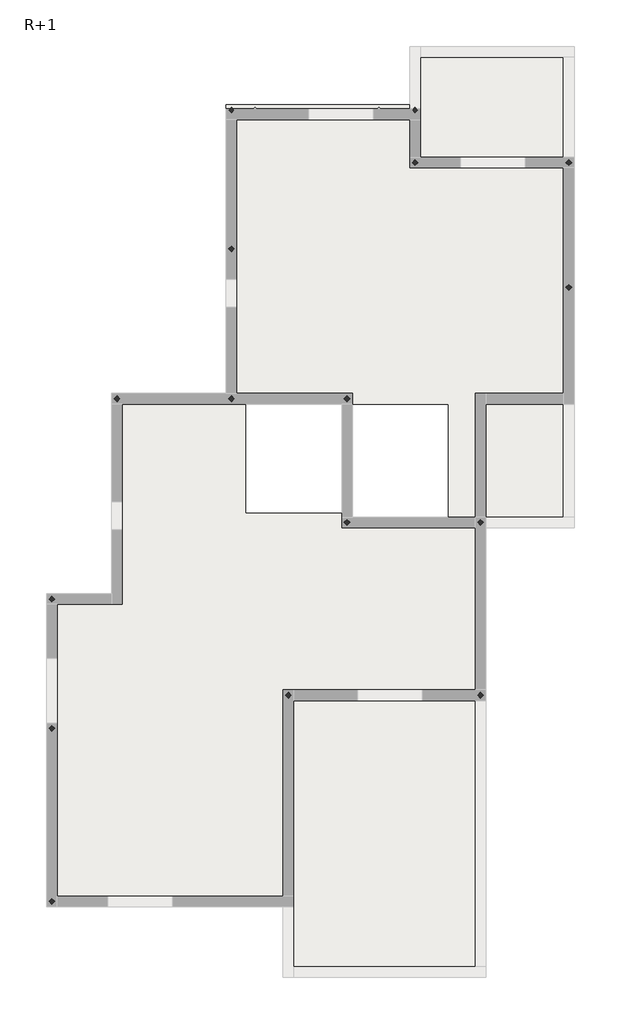
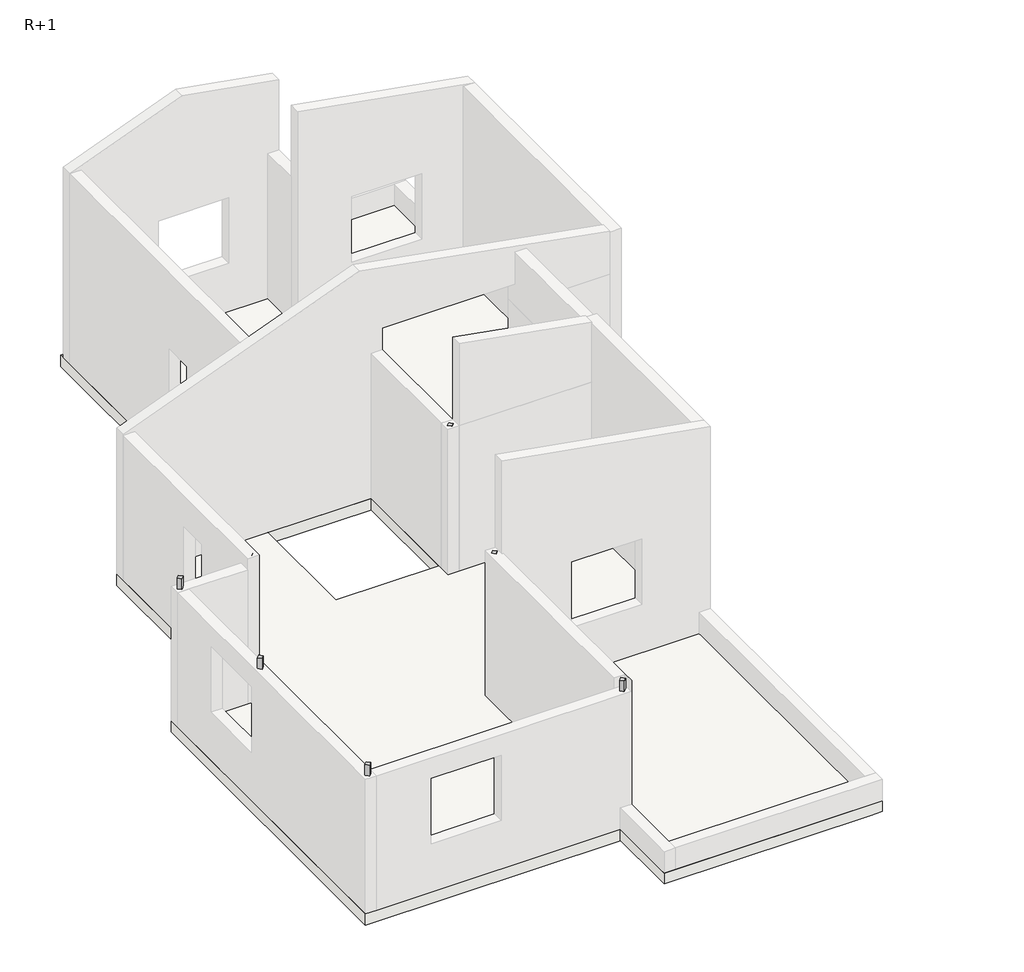
# One storey, part 2 of 2: 20 columns, 4 slabs, 1 beam.
"""IFC4 building model written with IfcOpenShell, lengths in millimetres."""

import ifcopenshell
import ifcopenshell.guid

model = None  # the IFC model being written
_history = None  # IfcOwnerHistory: only IFC2X3 demands one
_inside = {}  # id of a spatial element -> (the spatial element, [elements in it])
_under = {}  # id of a project, library or spatial element -> (it, [spatial elements below it])
_declared = {}  # id of a project -> (the project, [libraries it declares])
_typed = {}  # id of a type object -> (the type object, [elements of that type])
_made_of = {}  # id of a material, layer set ... -> (it, [elements and type objects made of it])


def new_model(schema):
    """Start an empty IFC model of exactly this schema.

    Asked for "IFC4X3", IfcOpenShell would pick the latest addendum, in which some entities
    have other attributes; the version numbers below select the first issue.
    IFC2X3 requires an IfcOwnerHistory on every rooted entity: one is made here for all.
    """
    global model, _history
    if schema == "IFC4X3":
        model = ifcopenshell.file(schema_version=(4, 3, 0, 0))
    else:
        model = ifcopenshell.file(schema=schema)
    _inside.clear()
    _under.clear()
    _declared.clear()
    _typed.clear()
    _made_of.clear()
    _history = None
    if model.schema == "IFC2X3":
        org = make("IfcOrganization", Name="unknown")
        user = make(
            "IfcPersonAndOrganization",
            ThePerson=make("IfcPerson", FamilyName="unknown"),
            TheOrganization=org,
        )
        app = make(
            "IfcApplication",
            ApplicationDeveloper=org,
            Version="unknown",
            ApplicationFullName="unknown",
            ApplicationIdentifier="unknown",
        )
        _history = make(
            "IfcOwnerHistory",
            OwningUser=user,
            OwningApplication=app,
            ChangeAction="ADDED",
            CreationDate=0,
        )
    return model


def make(cls, **values):
    """One entity of the class cls with the attributes given. An attribute that is None is left unset."""
    return model.create_entity(
        cls, **{name: value for name, value in values.items() if value is not None}
    )


def rooted(cls, **values):
    """An entity with a GlobalId (a new one), such as an element, a storey or a relation."""
    return make(cls, GlobalId=ifcopenshell.guid.new(), OwnerHistory=_history, **values)


def si_unit(unit_type, name, prefix=None):
    """IfcSIUnit, for example si_unit("LENGTHUNIT", "METRE", prefix="MILLI")."""
    return make("IfcSIUnit", UnitType=unit_type, Prefix=prefix, Name=name)


def assignment(units):
    """IfcUnitAssignment: the units of a project."""
    return None if units is None else make("IfcUnitAssignment", Units=units)


def point(xyz):
    """IfcCartesianPoint."""
    return None if xyz is None else make("IfcCartesianPoint", Coordinates=xyz)


def direction(xyz):
    """IfcDirection."""
    return None if xyz is None else make("IfcDirection", DirectionRatios=xyz)


def frame(location, z_axis=None, x_axis=None):
    """IfcAxis2Placement3D, a coordinate frame: its origin and axes. An axis left out is left unset."""
    return make(
        "IfcAxis2Placement3D",
        Location=point(location),
        Axis=direction(z_axis),
        RefDirection=direction(x_axis),
    )


def origin():
    """The frame at (0, 0, 0) with its axes left unset."""
    return frame((0.0, 0.0, 0.0))


def place(relative_to, where):
    """IfcLocalPlacement: puts the frame where relative to a parent placement (None: the world)."""
    return make(
        "IfcLocalPlacement", PlacementRelTo=relative_to, RelativePlacement=where
    )


def context(
    kind, dimensions, precision=None, world=None, true_north=None, identifier=None
):
    """IfcGeometricRepresentationContext, for example the 3D "Model" context."""
    return make(
        "IfcGeometricRepresentationContext",
        ContextIdentifier=identifier,
        ContextType=kind,
        CoordinateSpaceDimension=dimensions,
        Precision=precision,
        WorldCoordinateSystem=world,
        TrueNorth=true_north,
    )


def project(units=None, contexts=None):
    """IfcProject with its units and contexts."""
    return rooted(
        "IfcProject",
        Name="project",
        RepresentationContexts=contexts,
        UnitsInContext=assignment(units),
    )


def spatial(cls, under=None, at=None, **own):
    """A site, building, storey or space (cls), placed at a placement, below another one or the project."""
    s = rooted(cls, ObjectPlacement=at, **own)
    if under is not None:
        _under.setdefault(under.id(), (under, []))[1].append(s)
    return s


def polyline(points):
    """IfcPolyline through the points."""
    return make("IfcPolyline", Points=[point(p) for p in points])


def outline(outer, holes=None, kind="AREA"):
    """IfcArbitraryClosedProfileDef: a profile drawn as a closed curve; with holes, ...WithVoids."""
    if holes is None:
        return make("IfcArbitraryClosedProfileDef", ProfileType=kind, OuterCurve=outer)
    return make(
        "IfcArbitraryProfileDefWithVoids",
        ProfileType=kind,
        OuterCurve=outer,
        InnerCurves=holes,
    )


def extrude(swept, where, along, depth):
    """IfcExtrudedAreaSolid: the profile swept, set in the frame where, extruded along a direction by depth."""
    return make(
        "IfcExtrudedAreaSolid",
        SweptArea=swept,
        Position=where,
        ExtrudedDirection=direction(along),
        Depth=depth,
    )


def faces_of(points, faces, orient=None, outer=None):
    """IfcFace entities. A face is a list of loops; a loop is a list of indices into points, from 0.

    orient and outer hold one flag for each loop. By default every Orientation is true, the
    first loop of a face is its IfcFaceOuterBound and the others are IfcFaceBound.
    """
    made = []
    for i, loops in enumerate(faces):
        bounds = []
        for j, loop in enumerate(loops):
            is_outer = j == 0 if outer is None else outer[i][j]
            bounds.append(
                make(
                    "IfcFaceOuterBound" if is_outer else "IfcFaceBound",
                    Bound=make("IfcPolyLoop", Polygon=[points[k] for k in loop]),
                    Orientation=True if orient is None else orient[i][j],
                )
            )
        made.append(make("IfcFace", Bounds=bounds))
    return made


def faceted_brep(points, faces, orient=None, outer=None, voids=None):
    """IfcFacetedBrep: a solid bounded by flat faces; with voids (closed shells), ...WithVoids."""
    shared = [point(p) for p in points]
    hull = make("IfcClosedShell", CfsFaces=faces_of(shared, faces, orient, outer))
    if voids is None:
        return make("IfcFacetedBrep", Outer=hull)
    return make(
        "IfcFacetedBrepWithVoids",
        Outer=hull,
        Voids=[
            make(cls, CfsFaces=faces_of(shared, fs, o, b)) for cls, fs, o, b in voids
        ],
    )


def shape(context_of_items, identifier, shape_type, items):
    """IfcShapeRepresentation: the items that make up one representation, for example the "Body"."""
    return make(
        "IfcShapeRepresentation",
        ContextOfItems=context_of_items,
        RepresentationIdentifier=identifier,
        RepresentationType=shape_type,
        Items=items,
    )


def made_of(thing, what):
    """Note that an element or type object is made of a material, layer set ...; save() writes the relation."""
    if what is not None:
        _made_of.setdefault(what.id(), (what, []))[1].append(thing)
    return thing


def element(
    cls,
    number,
    at=None,
    inside=None,
    cuts=None,
    type_object=None,
    material=None,
    context=None,
    identifier="Body",
    shape_type=None,
    held_by="IfcProductDefinitionShape",
    body=None,
    shapes=None,
    **own,
):
    """One element of the class cls, such as IfcWall. Its Tag is "e" and its number.

    at: its placement. inside: the storey or other place that contains it. cuts: it is an
    opening in that element (IfcRelVoidsElement). A single representation is given by context,
    identifier, shape_type and body (its items); several are given by shapes. held_by: the class
    of the entity that holds the representations. save() writes the other relations.
    """
    e = rooted(cls, Tag="e%d" % number, ObjectPlacement=at, **own)
    if body is not None:
        shapes = [shape(context, identifier, shape_type, body)]
    if shapes is not None:
        e.Representation = make(held_by, Representations=shapes)
    if inside is not None:
        _inside.setdefault(inside.id(), (inside, []))[1].append(e)
    if cuts is not None:
        rooted(
            "IfcRelVoidsElement", RelatingBuildingElement=cuts, RelatedOpeningElement=e
        )
    if type_object is not None:
        _typed.setdefault(type_object.id(), (type_object, []))[1].append(e)
    return made_of(e, material)


def aggregate(whole, parts):
    """IfcRelAggregates: a whole, such as a stair, and the parts it consists of."""
    return rooted("IfcRelAggregates", RelatingObject=whole, RelatedObjects=parts)


def save(model, path):
    """Write the relations noted so far, then the file.

    IfcRelAggregates (storeys below a building ...), IfcRelContainedInSpatialStructure (elements
    in a storey), IfcRelDefinesByType, IfcRelAssociatesMaterial and IfcRelDeclares: one each for
    every whole, place, type object, material and project.
    """
    for whole, parts in _under.values():
        aggregate(whole, parts)
    for where, things in _inside.values():
        rooted(
            "IfcRelContainedInSpatialStructure",
            RelatedElements=things,
            RelatingStructure=where,
        )
    for kind, things in _typed.values():
        rooted("IfcRelDefinesByType", RelatedObjects=things, RelatingType=kind)
    for what, things in _made_of.values():
        rooted("IfcRelAssociatesMaterial", RelatedObjects=things, RelatingMaterial=what)
    for by, libraries in _declared.values():
        rooted("IfcRelDeclares", RelatingContext=by, RelatedDefinitions=libraries)
    model.write(path)


model = new_model("IFC4")

# Units and contexts
model_context = context("Model", 3, world=origin())
ifc_project = project(units=[si_unit("LENGTHUNIT", "METRE", prefix="MILLI")], contexts=[model_context])

# Site, building, storey
site = spatial("IfcSite", under=ifc_project)
building = spatial("IfcBuilding", under=site)
storey = spatial("IfcBuildingStorey", under=building, Name="R+1", Elevation=2710.0)

# Beam
placement = place(None, origin())
element("IfcBeam", 1, ObjectType="Poutres BA : 20x30ht", at=placement, inside=storey, context=model_context, shape_type="SweptSolid", body=[
    extrude(outline(polyline([(-2475.4327864, 897.5075352), (-2675.4327864, 897.5075352), (-2675.4327864, 2763.8353669), (-2475.4327864, 2763.8353669), (-2475.4327864, 897.5075352)])), frame((0.0, 0.0, 2400.0), z_axis=(0.0, 0.0, 1.0), x_axis=(1.0, 0.0, 0.0)), (0.0, 0.0, 1.0), 100.0),
])

# Columns
element("IfcColumn", 2, ObjectType="CV : CV", at=placement, inside=storey, context=model_context, shape_type="SweptSolid", body=[
    extrude(outline(polyline([(-4912.6214092, 2916.8683755), (-4859.5884006, 2863.8353669), (-4912.6214092, 2810.8023583), (-4965.6544178, 2863.8353669), (-4912.6214092, 2916.8683755)])), frame((0.0, 0.0, 2710.0), z_axis=(0.0, 0.0, 1.0), x_axis=(1.0, 0.0, 0.0)), (0.0, 0.0, 1.0), 2700.0),
    extrude(outline(polyline([(-4859.5884006, 2863.8353669), (-4912.6214092, 2810.8023583), (-4965.6544178, 2863.8353669), (-4912.6214092, 2916.8683755), (-4859.5884006, 2863.8353669)])), frame((0.0, 0.0, 2710.0), z_axis=(0.0, 0.0, 1.0), x_axis=(1.0, 0.0, 0.0)), (0.0, 0.0, 1.0), 2700.0),
])
element("IfcColumn", 3, ObjectType="CV : CV", at=placement, inside=storey, context=model_context, shape_type="SweptSolid", body=[
    extrude(outline(polyline([(-2745.4336004, 2916.8683755), (-2692.4005918, 2863.8353669), (-2745.4336004, 2810.8023583), (-2798.466609, 2863.8353669), (-2745.4336004, 2916.8683755)])), frame((0.0, 0.0, 2710.0), z_axis=(0.0, 0.0, 1.0), x_axis=(1.0, 0.0, 0.0)), (0.0, 0.0, 1.0), 2700.0),
    extrude(outline(polyline([(-2692.4005918, 2863.8353669), (-2745.4336004, 2810.8023583), (-2798.466609, 2863.8353669), (-2745.4336004, 2916.8683755), (-2692.4005918, 2863.8353669)])), frame((0.0, 0.0, 2710.0), z_axis=(0.0, 0.0, 1.0), x_axis=(1.0, 0.0, 0.0)), (0.0, 0.0, 1.0), 2700.0),
])
element("IfcColumn", 4, ObjectType="CV : CV", at=placement, inside=storey, context=model_context, shape_type="SweptSolid", body=[
    extrude(outline(polyline([(-2745.4336004, 5751.8684051), (-2692.4005918, 5698.8353965), (-2745.4336004, 5645.8023879), (-2798.466609, 5698.8353965), (-2745.4336004, 5751.8684051)])), frame((0.0, 0.0, 2710.0), z_axis=(0.0, 0.0, 1.0), x_axis=(1.0, 0.0, 0.0)), (0.0, 0.0, 1.0), 2700.0),
    extrude(outline(polyline([(-2692.4005918, 5698.8353965), (-2745.4336004, 5645.8023879), (-2798.466609, 5698.8353965), (-2745.4336004, 5751.8684051), (-2692.4005918, 5698.8353965)])), frame((0.0, 0.0, 2710.0), z_axis=(0.0, 0.0, 1.0), x_axis=(1.0, 0.0, 0.0)), (0.0, 0.0, 1.0), 2700.0),
])
element("IfcColumn", 5, ObjectType="CV : CV", at=placement, inside=storey, context=model_context, shape_type="Brep", body=[
    faceted_brep([(-2745.4336004, 8376.8684051, 5410.0), (-2774.0361474, 8348.2658581, 5410.0), (-2798.466609, 8323.8353965, 5410.0), (-2745.4336004, 8270.8023879, 5410.0), (-2692.4005918, 8323.8353965, 5410.0), (-2716.8310535, 8348.2658581, 5410.0), (-2745.4336004, 8376.8684051, 2710.0), (-2716.8310535, 8348.2658581, 2710.0), (-2692.4005918, 8323.8353965, 2710.0), (-2745.4336004, 8270.8023879, 2710.0), (-2798.466609, 8323.8353965, 2710.0), (-2774.0361474, 8348.2658581, 2710.0)], [[[0, 1, 2, 3, 4, 5]], [[6, 7, 8, 9, 10, 11]], [[2, 1, 0, 6, 11, 10]], [[3, 2, 10, 9]], [[4, 3, 9, 8]], [[0, 5, 4, 8, 7, 6]]]),
    faceted_brep([(-2692.4005918, 8323.8353965, 5410.0), (-2716.8310535, 8348.2658581, 5410.0), (-2745.4336004, 8376.8684051, 5410.0), (-2774.0361474, 8348.2658581, 5410.0), (-2798.466609, 8323.8353965, 5410.0), (-2745.4336004, 8270.8023879, 5410.0), (-2692.4005918, 8323.8353965, 2710.0), (-2745.4336004, 8270.8023879, 2710.0), (-2798.466609, 8323.8353965, 2710.0), (-2774.0361474, 8348.2658581, 2710.0), (-2745.4336004, 8376.8684051, 2710.0), (-2716.8310535, 8348.2658581, 2710.0)], [[[0, 1, 2, 3, 4, 5]], [[6, 7, 8, 9, 10, 11]], [[2, 1, 0, 6, 11, 10]], [[4, 3, 2, 10, 9, 8]], [[5, 4, 8, 7]], [[0, 5, 7, 6]]]),
])
element("IfcColumn", 6, ObjectType="CV : CV", at=placement, inside=storey, context=model_context, shape_type="Brep", body=[
    faceted_brep([(734.5663791, 8376.8684051, 5410.0), (705.9638322, 8348.2658581, 5410.0), (681.5333706, 8323.8353965, 5410.0), (734.5663791, 8270.8023879, 5410.0), (787.5993877, 8323.8353965, 5410.0), (763.1689261, 8348.2658581, 5410.0), (734.5663791, 8376.8684051, 2710.0), (763.1689261, 8348.2658581, 2710.0), (787.5993877, 8323.8353965, 2710.0), (734.5663791, 8270.8023879, 2710.0), (681.5333706, 8323.8353965, 2710.0), (705.9638322, 8348.2658581, 2710.0)], [[[0, 1, 2, 3, 4, 5]], [[6, 7, 8, 9, 10, 11]], [[2, 1, 0, 6, 11, 10]], [[3, 2, 10, 9]], [[4, 3, 9, 8]], [[0, 5, 4, 8, 7, 6]]]),
    faceted_brep([(787.5993877, 8323.8353965, 5410.0), (763.1689261, 8348.2658581, 5410.0), (734.5663791, 8376.8684051, 5410.0), (705.9638322, 8348.2658581, 5410.0), (681.5333706, 8323.8353965, 5410.0), (734.5663791, 8270.8023879, 5410.0), (787.5993877, 8323.8353965, 2710.0), (734.5663791, 8270.8023879, 2710.0), (681.5333706, 8323.8353965, 2710.0), (705.9638322, 8348.2658581, 2710.0), (734.5663791, 8376.8684051, 2710.0), (763.1689261, 8348.2658581, 2710.0)], [[[0, 1, 2, 3, 4, 5]], [[6, 7, 8, 9, 10, 11]], [[2, 1, 0, 6, 11, 10]], [[4, 3, 2, 10, 9, 8]], [[5, 4, 8, 7]], [[0, 5, 7, 6]]]),
])
element("IfcColumn", 7, ObjectType="CV : CV", at=placement, inside=storey, context=model_context, shape_type="SweptSolid", body=[
    extrude(outline(polyline([(734.5663791, 7386.0121016), (787.5993877, 7332.979093), (734.5663791, 7279.9460844), (681.5333706, 7332.979093), (734.5663791, 7386.0121016)])), frame((0.0, 0.0, 2710.0), z_axis=(0.0, 0.0, 1.0), x_axis=(1.0, 0.0, 0.0)), (0.0, 0.0, 1.0), 2700.0),
    extrude(outline(polyline([(787.5993877, 7332.979093), (734.5663791, 7279.9460844), (681.5333706, 7332.979093), (734.5663791, 7386.0121016), (787.5993877, 7332.979093)])), frame((0.0, 0.0, 2710.0), z_axis=(0.0, 0.0, 1.0), x_axis=(1.0, 0.0, 0.0)), (0.0, 0.0, 1.0), 2700.0),
])
element("IfcColumn", 8, ObjectType="CV : CV", at=placement, inside=storey, context=model_context, shape_type="SweptSolid", body=[
    extrude(outline(polyline([(3644.5663998, 7386.0121016), (3697.5994084, 7332.979093), (3644.5663998, 7279.9460844), (3591.5333912, 7332.979093), (3644.5663998, 7386.0121016)])), frame((0.0, 0.0, 2710.0), z_axis=(0.0, 0.0, 1.0), x_axis=(1.0, 0.0, 0.0)), (0.0, 0.0, 1.0), 2700.0),
    extrude(outline(polyline([(3697.5994084, 7332.979093), (3644.5663998, 7279.9460844), (3591.5333912, 7332.979093), (3644.5663998, 7386.0121016), (3697.5994084, 7332.979093)])), frame((0.0, 0.0, 2710.0), z_axis=(0.0, 0.0, 1.0), x_axis=(1.0, 0.0, 0.0)), (0.0, 0.0, 1.0), 2700.0),
])
element("IfcColumn", 9, ObjectType="CV : CV", at=placement, inside=storey, context=model_context, shape_type="SweptSolid", body=[
    extrude(outline(polyline([(3644.5663998, 5026.0121016), (3697.5994084, 4972.979093), (3644.5663998, 4919.9460844), (3591.5333912, 4972.979093), (3644.5663998, 5026.0121016)])), frame((0.0, 0.0, 2710.0), z_axis=(0.0, 0.0, 1.0), x_axis=(1.0, 0.0, 0.0)), (0.0, 0.0, 1.0), 2700.0),
    extrude(outline(polyline([(3697.5994084, 4972.979093), (3644.5663998, 4919.9460844), (3591.5333912, 4972.979093), (3644.5663998, 5026.0121016), (3697.5994084, 4972.979093)])), frame((0.0, 0.0, 2710.0), z_axis=(0.0, 0.0, 1.0), x_axis=(1.0, 0.0, 0.0)), (0.0, 0.0, 1.0), 2700.0),
])
element("IfcColumn", 10, ObjectType="CV : CV", at=placement, inside=storey, context=model_context, shape_type="SweptSolid", body=[
    extrude(outline(polyline([(3644.5663998, 2916.8683755), (3697.5994084, 2863.8353669), (3644.5663998, 2810.8023583), (3591.5333912, 2863.8353669), (3644.5663998, 2916.8683755)])), frame((0.0, 0.0, 2710.0), z_axis=(0.0, 0.0, 1.0), x_axis=(1.0, 0.0, 0.0)), (0.0, 0.0, 1.0), 2700.0),
    extrude(outline(polyline([(3697.5994084, 2863.8353669), (3644.5663998, 2810.8023583), (3591.5333912, 2863.8353669), (3644.5663998, 2916.8683755), (3697.5994084, 2863.8353669)])), frame((0.0, 0.0, 2710.0), z_axis=(0.0, 0.0, 1.0), x_axis=(1.0, 0.0, 0.0)), (0.0, 0.0, 1.0), 2700.0),
])
element("IfcColumn", 11, ObjectType="CV : CV", at=placement, inside=storey, context=model_context, shape_type="SweptSolid", body=[
    extrude(outline(polyline([(1974.5663639, 2916.8683755), (2027.5993725, 2863.8353669), (1974.5663639, 2810.8023583), (1921.5333553, 2863.8353669), (1974.5663639, 2916.8683755)])), frame((0.0, 0.0, 2710.0), z_axis=(0.0, 0.0, 1.0), x_axis=(1.0, 0.0, 0.0)), (0.0, 0.0, 1.0), 2700.0),
    extrude(outline(polyline([(2027.5993725, 2863.8353669), (1974.5663639, 2810.8023583), (1921.5333553, 2863.8353669), (1974.5663639, 2916.8683755), (2027.5993725, 2863.8353669)])), frame((0.0, 0.0, 2710.0), z_axis=(0.0, 0.0, 1.0), x_axis=(1.0, 0.0, 0.0)), (0.0, 0.0, 1.0), 2700.0),
])
element("IfcColumn", 12, ObjectType="CV : CV", at=placement, inside=storey, context=model_context, shape_type="SweptSolid", body=[
    extrude(outline(polyline([(1974.5663639, 576.8683759), (2027.5993725, 523.8353673), (1974.5663639, 470.8023588), (1921.5333553, 523.8353673), (1974.5663639, 576.8683759)])), frame((0.0, 0.0, 2710.0), z_axis=(0.0, 0.0, 1.0), x_axis=(1.0, 0.0, 0.0)), (0.0, 0.0, 1.0), 2700.0),
    extrude(outline(polyline([(2027.5993725, 523.8353673), (1974.5663639, 470.8023588), (1921.5333553, 523.8353673), (1974.5663639, 576.8683759), (2027.5993725, 523.8353673)])), frame((0.0, 0.0, 2710.0), z_axis=(0.0, 0.0, 1.0), x_axis=(1.0, 0.0, 0.0)), (0.0, 0.0, 1.0), 2700.0),
])
element("IfcColumn", 13, ObjectType="CV : CV", at=placement, inside=storey, context=model_context, shape_type="SweptSolid", body=[
    extrude(outline(polyline([(1974.5663639, -2693.1316224), (2027.5993725, -2746.164631), (1974.5663639, -2799.1976396), (1921.5333553, -2746.164631), (1974.5663639, -2693.1316224)])), frame((0.0, 0.0, 2710.0), z_axis=(0.0, 0.0, 1.0), x_axis=(1.0, 0.0, 0.0)), (0.0, 0.0, 1.0), 2700.0),
    extrude(outline(polyline([(2027.5993725, -2746.164631), (1974.5663639, -2799.1976396), (1921.5333553, -2746.164631), (1974.5663639, -2693.1316224), (2027.5993725, -2746.164631)])), frame((0.0, 0.0, 2710.0), z_axis=(0.0, 0.0, 1.0), x_axis=(1.0, 0.0, 0.0)), (0.0, 0.0, 1.0), 2700.0),
])
element("IfcColumn", 14, ObjectType="CV : CV", at=placement, inside=storey, context=model_context, shape_type="SweptSolid", body=[
    extrude(outline(polyline([(-1666.4904447, -2693.1316224), (-1613.4574361, -2746.164631), (-1666.4904447, -2799.1976396), (-1719.5234533, -2746.164631), (-1666.4904447, -2693.1316224)])), frame((0.0, 0.0, 2710.0), z_axis=(0.0, 0.0, 1.0), x_axis=(1.0, 0.0, 0.0)), (0.0, 0.0, 1.0), 2700.0),
    extrude(outline(polyline([(-1613.4574361, -2746.164631), (-1666.4904447, -2799.1976396), (-1719.5234533, -2746.164631), (-1666.4904447, -2693.1316224), (-1613.4574361, -2746.164631)])), frame((0.0, 0.0, 2710.0), z_axis=(0.0, 0.0, 1.0), x_axis=(1.0, 0.0, 0.0)), (0.0, 0.0, 1.0), 2700.0),
])
element("IfcColumn", 15, ObjectType="CV : CV", at=placement, inside=storey, context=model_context, shape_type="SweptSolid", body=[
    extrude(outline(polyline([(-1666.4904447, -6595.6690755), (-1613.4574361, -6648.7020841), (-1666.4904447, -6701.7350927), (-1719.5234533, -6648.7020841), (-1666.4904447, -6595.6690755)])), frame((0.0, 0.0, 2710.0), z_axis=(0.0, 0.0, 1.0), x_axis=(1.0, 0.0, 0.0)), (0.0, 0.0, 1.0), 2700.0),
    extrude(outline(polyline([(-1613.4574361, -6648.7020841), (-1666.4904447, -6701.7350927), (-1719.5234533, -6648.7020841), (-1666.4904447, -6595.6690755), (-1613.4574361, -6648.7020841)])), frame((0.0, 0.0, 2710.0), z_axis=(0.0, 0.0, 1.0), x_axis=(1.0, 0.0, 0.0)), (0.0, 0.0, 1.0), 2700.0),
])
element("IfcColumn", 16, ObjectType="CV : CV", at=placement, inside=storey, context=model_context, shape_type="Brep", body=[
    faceted_brep([(-6146.4904447, -6595.6690755, 5410.0), (-6199.5234533, -6648.7020841, 5410.0), (-6146.4904447, -6701.7350927, 5410.0), (-6093.4574361, -6648.7020841, 5410.0), (-6146.4904447, -6595.6690755, 2710.0), (-6093.4574361, -6648.7020841, 2710.0), (-6146.4904447, -6701.7350927, 2710.0), (-6199.5234533, -6648.7020841, 2710.0), (-6146.4904447, -6595.6690755, 5210.0), (-6199.5234533, -6648.7020841, 5210.0), (-6146.4904447, -6701.7350927, 5210.0), (-6093.4574361, -6648.7020841, 5210.0)], [[[0, 1, 2, 3]], [[4, 5, 6, 7]], [[1, 0, 8, 4, 7, 9]], [[2, 1, 9, 7, 6, 10]], [[3, 2, 10, 6, 5, 11]], [[0, 3, 11, 5, 4, 8]]]),
    faceted_brep([(-6093.4574361, -6648.7020841, 5410.0), (-6146.4904447, -6595.6690755, 5410.0), (-6199.5234533, -6648.7020841, 5410.0), (-6146.4904447, -6701.7350927, 5410.0), (-6093.4574361, -6648.7020841, 2710.0), (-6146.4904447, -6701.7350927, 2710.0), (-6199.5234533, -6648.7020841, 2710.0), (-6146.4904447, -6595.6690755, 2710.0), (-6093.4574361, -6648.7020841, 5210.0), (-6146.4904447, -6595.6690755, 5210.0), (-6199.5234533, -6648.7020841, 5210.0), (-6146.4904447, -6701.7350927, 5210.0)], [[[0, 1, 2, 3]], [[4, 5, 6, 7]], [[1, 0, 8, 4, 7, 9]], [[2, 1, 9, 7, 6, 10]], [[3, 2, 10, 6, 5, 11]], [[0, 3, 11, 5, 4, 8]]]),
])
element("IfcColumn", 17, ObjectType="CV : CV", at=placement, inside=storey, context=model_context, shape_type="Brep", body=[
    faceted_brep([(-6146.4904447, -3320.527527, 5410.0), (-6199.5234533, -3373.5605356, 5410.0), (-6146.4904447, -3426.5935442, 5410.0), (-6093.4574361, -3373.5605356, 5410.0), (-6146.4904447, -3320.527527, 2710.0), (-6093.4574361, -3373.5605356, 2710.0), (-6146.4904447, -3426.5935442, 2710.0), (-6199.5234533, -3373.5605356, 2710.0), (-6146.4904447, -3320.527527, 5210.0), (-6199.5234533, -3373.5605356, 5210.0), (-6146.4904447, -3426.5935442, 5210.0), (-6093.4574361, -3373.5605356, 5210.0)], [[[0, 1, 2, 3]], [[4, 5, 6, 7]], [[1, 0, 8, 4, 7, 9]], [[2, 1, 9, 7, 6, 10]], [[3, 2, 10, 6, 5, 11]], [[0, 3, 11, 5, 4, 8]]]),
    faceted_brep([(-6093.4574361, -3373.5605356, 5410.0), (-6146.4904447, -3320.527527, 5410.0), (-6199.5234533, -3373.5605356, 5410.0), (-6146.4904447, -3426.5935442, 5410.0), (-6093.4574361, -3373.5605356, 2710.0), (-6146.4904447, -3426.5935442, 2710.0), (-6199.5234533, -3373.5605356, 2710.0), (-6146.4904447, -3320.527527, 2710.0), (-6093.4574361, -3373.5605356, 5210.0), (-6146.4904447, -3320.527527, 5210.0), (-6199.5234533, -3373.5605356, 5210.0), (-6146.4904447, -3426.5935442, 5210.0)], [[[0, 1, 2, 3]], [[4, 5, 6, 7]], [[1, 0, 8, 4, 7, 9]], [[2, 1, 9, 7, 6, 10]], [[3, 2, 10, 6, 5, 11]], [[0, 3, 11, 5, 4, 8]]]),
])
element("IfcColumn", 18, ObjectType="CV : CV", at=placement, inside=storey, context=model_context, shape_type="Brep", body=[
    faceted_brep([(-6146.4904447, -875.527527, 5410.0), (-6199.5234533, -928.5605356, 5410.0), (-6146.4904447, -981.5935442, 5410.0), (-6093.4574361, -928.5605356, 5410.0), (-6146.4904447, -875.527527, 2710.0), (-6093.4574361, -928.5605356, 2710.0), (-6146.4904447, -981.5935442, 2710.0), (-6199.5234533, -928.5605356, 2710.0), (-6146.4904447, -875.527527, 5210.0), (-6199.5234533, -928.5605356, 5210.0), (-6146.4904447, -981.5935442, 5210.0), (-6093.4574361, -928.5605356, 5210.0)], [[[0, 1, 2, 3]], [[4, 5, 6, 7]], [[1, 0, 8, 4, 7, 9]], [[2, 1, 9, 7, 6, 10]], [[3, 2, 10, 6, 5, 11]], [[0, 3, 11, 5, 4, 8]]]),
    faceted_brep([(-6093.4574361, -928.5605356, 5410.0), (-6146.4904447, -875.527527, 5410.0), (-6199.5234533, -928.5605356, 5410.0), (-6146.4904447, -981.5935442, 5410.0), (-6093.4574361, -928.5605356, 2710.0), (-6146.4904447, -981.5935442, 2710.0), (-6199.5234533, -928.5605356, 2710.0), (-6146.4904447, -875.527527, 2710.0), (-6093.4574361, -928.5605356, 5210.0), (-6146.4904447, -875.527527, 5210.0), (-6199.5234533, -928.5605356, 5210.0), (-6146.4904447, -981.5935442, 5210.0)], [[[0, 1, 2, 3]], [[4, 5, 6, 7]], [[1, 0, 8, 4, 7, 9]], [[2, 1, 9, 7, 6, 10]], [[3, 2, 10, 6, 5, 11]], [[0, 3, 11, 5, 4, 8]]]),
])
element("IfcColumn", 19, ObjectType="CV : CV", at=placement, inside=storey, context=model_context, shape_type="SweptSolid", body=[
    extrude(outline(polyline([(-4912.6214092, -875.527527), (-4859.5884006, -928.5605356), (-4912.6214092, -981.5935442), (-4965.6544178, -928.5605356), (-4912.6214092, -875.527527)])), frame((0.0, 0.0, 2710.0), z_axis=(0.0, 0.0, 1.0), x_axis=(1.0, 0.0, 0.0)), (0.0, 0.0, 1.0), 2700.0),
    extrude(outline(polyline([(-4859.5884006, -928.5605356), (-4912.6214092, -981.5935442), (-4965.6544178, -928.5605356), (-4912.6214092, -875.527527), (-4859.5884006, -928.5605356)])), frame((0.0, 0.0, 2710.0), z_axis=(0.0, 0.0, 1.0), x_axis=(1.0, 0.0, 0.0)), (0.0, 0.0, 1.0), 2700.0),
])
element("IfcColumn", 20, ObjectType="CV : CV", at=placement, inside=storey, context=model_context, shape_type="SweptSolid", body=[
    extrude(outline(polyline([(-555.4335965, 2916.8683755), (-502.4005879, 2863.8353669), (-555.4335965, 2810.8023583), (-608.4666051, 2863.8353669), (-555.4335965, 2916.8683755)])), frame((0.0, 0.0, 2710.0), z_axis=(0.0, 0.0, 1.0), x_axis=(1.0, 0.0, 0.0)), (0.0, 0.0, 1.0), 2700.0),
    extrude(outline(polyline([(-502.4005879, 2863.8353669), (-555.4335965, 2810.8023583), (-608.4666051, 2863.8353669), (-555.4335965, 2916.8683755), (-502.4005879, 2863.8353669)])), frame((0.0, 0.0, 2710.0), z_axis=(0.0, 0.0, 1.0), x_axis=(1.0, 0.0, 0.0)), (0.0, 0.0, 1.0), 2700.0),
])
element("IfcColumn", 21, ObjectType="CV : CV", at=placement, inside=storey, context=model_context, shape_type="SweptSolid", body=[
    extrude(outline(polyline([(-555.4335965, 576.8683759), (-502.4005879, 523.8353673), (-555.4335965, 470.8023588), (-608.4666051, 523.8353673), (-555.4335965, 576.8683759)])), frame((0.0, 0.0, 2710.0), z_axis=(0.0, 0.0, 1.0), x_axis=(1.0, 0.0, 0.0)), (0.0, 0.0, 1.0), 2700.0),
    extrude(outline(polyline([(-502.4005879, 523.8353673), (-555.4335965, 470.8023588), (-608.4666051, 523.8353673), (-555.4335965, 576.8683759), (-502.4005879, 523.8353673)])), frame((0.0, 0.0, 2710.0), z_axis=(0.0, 0.0, 1.0), x_axis=(1.0, 0.0, 0.0)), (0.0, 0.0, 1.0), 2700.0),
])

# Slabs
element("IfcSlab", 22, ObjectType="Dalla BA 20", at=placement, inside=storey, context=model_context, shape_type="Brep", body=[
    faceted_brep([(2074.5663809, -8086.16463, 2510.0), (1874.5663809, -8086.16463, 2510.0), (-1766.4904447, -8086.16463, 2510.0), (-1766.4904447, -7886.16463, 2510.0), (-1766.4904447, -6748.702077, 2510.0), (-1566.4904447, -6748.702077, 2510.0), (-1566.4904447, -2846.1646234, 2510.0), (1874.5663809, -2846.1646234, 2510.0), (2074.5663809, -2846.1646234, 2510.0), (2027.5993725, -5366.1646244, 2510.0), (1974.5663639, -5313.1316158, 2510.0), (1921.5333553, -5366.1646244, 2510.0), (1974.5663639, -5419.197633, 2510.0), (-802.4006105, -7986.1646298, 2510.0), (-855.4336191, -7933.1316212, 2510.0), (-908.4666277, -7986.1646298, 2510.0), (-855.4336191, -8039.1976384, 2510.0), (-1612.400632, -7986.1646298, 2510.0), (-1665.4336406, -7933.1316212, 2510.0), (-1718.4666492, -7986.1646298, 2510.0), (-1665.4336406, -8039.1976384, 2510.0), (-1766.4904447, -8086.16463, 2710.0), (2074.5663809, -8086.16463, 2710.0), (2074.5663809, -2846.1646234, 2710.0), (-1566.4904447, -2846.1646234, 2710.0), (-1566.4904447, -6748.702077, 2710.0), (-1766.4904447, -6748.702077, 2710.0), (-855.4336191, -7933.1316212, 2710.0), (-802.4006105, -7986.1646298, 2710.0), (-855.4336191, -8039.1976384, 2710.0), (-908.4666277, -7986.1646298, 2710.0), (-1665.4336406, -7933.1316212, 2710.0), (-1612.400632, -7986.1646298, 2710.0), (-1665.4336406, -8039.1976384, 2710.0), (-1718.4666492, -7986.1646298, 2710.0), (1974.5663639, -5313.1316158, 2710.0), (2027.5993725, -5366.1646244, 2710.0), (1974.5663639, -5419.197633, 2710.0), (1921.5333553, -5366.1646244, 2710.0)], [[[0, 1, 2, 3, 4, 5, 6, 7, 8], [9, 10, 11, 12], [13, 14, 15, 16], [17, 18, 19, 20]], [[21, 22, 23, 24, 25, 26], [27, 28, 29, 30], [31, 32, 33, 34], [35, 36, 37, 38]], [[2, 1, 0, 22, 21]], [[2, 21, 26, 4, 3]], [[22, 0, 8, 23]], [[6, 24, 23, 8, 7]], [[24, 6, 5, 25]], [[25, 5, 4, 26]], [[13, 28, 27, 14]], [[14, 27, 30, 15]], [[15, 30, 29, 16]], [[28, 13, 16, 29]], [[17, 32, 31, 18]], [[18, 31, 34, 19]], [[19, 34, 33, 20]], [[32, 17, 20, 33]], [[9, 36, 35, 10]], [[10, 35, 38, 11]], [[11, 38, 37, 12]], [[36, 9, 12, 37]]]),
    faceted_brep([(3744.5663998, 7232.9791151, 2510.0), (3544.5663998, 7232.9791151, 2510.0), (634.5663962, 7232.9791151, 2510.0), (634.5663962, 8223.8353965, 2510.0), (634.5663962, 8423.8353965, 2510.0), (634.5663962, 9529.3149644, 2510.0), (834.5663962, 9529.3149644, 2510.0), (3744.5663998, 9529.3149644, 2510.0), (3744.5663998, 9329.3149644, 2510.0), (3697.5994084, 9429.3149644, 2510.0), (3644.5663998, 9482.347973, 2510.0), (3591.5333912, 9429.3149644, 2510.0), (3644.5663998, 9376.2819558, 2510.0), (787.5993877, 8323.8353965, 2510.0), (734.5663791, 8376.8684051, 2510.0), (681.5333706, 8323.8353965, 2510.0), (734.5663791, 8270.8023879, 2510.0), (787.5993877, 9429.3149644, 2510.0), (734.5663791, 9482.347973, 2510.0), (681.5333706, 9429.3149644, 2510.0), (734.5663791, 9376.2819558, 2510.0), (634.5663962, 7232.9791151, 2710.0), (3744.5663998, 7232.9791151, 2710.0), (3744.5663998, 7432.979093, 2710.0), (3744.5663998, 9529.3149644, 2710.0), (634.5663962, 9529.3149644, 2710.0), (634.5663962, 8423.8353965, 2710.0), (734.5663791, 9482.347973, 2710.0), (787.5993877, 9429.3149644, 2710.0), (734.5663791, 9376.2819558, 2710.0), (681.5333706, 9429.3149644, 2710.0), (3644.5663998, 9482.347973, 2710.0), (3697.5994084, 9429.3149644, 2710.0), (3644.5663998, 9376.2819558, 2710.0), (3591.5333912, 9429.3149644, 2710.0), (734.5663791, 8376.8684051, 2710.0), (763.1689261, 8348.2658581, 2710.0), (787.5993877, 8323.8353965, 2710.0), (734.5663791, 8270.8023879, 2710.0), (681.5333706, 8323.8353965, 2710.0), (705.9638322, 8348.2658581, 2710.0)], [[[0, 1, 2, 3, 4, 5, 6, 7, 8], [9, 10, 11, 12], [13, 14, 15, 16], [17, 18, 19, 20]], [[21, 22, 23, 24, 25, 26], [27, 28, 29, 30], [31, 32, 33, 34], [35, 36, 37, 38, 39, 40]], [[2, 1, 0, 22, 21]], [[2, 21, 26, 25, 5, 4, 3]], [[7, 6, 5, 25, 24]], [[0, 8, 7, 24, 23, 22]], [[13, 37, 36, 35, 14]], [[14, 35, 40, 39, 15]], [[15, 39, 38, 16]], [[37, 13, 16, 38]], [[17, 28, 27, 18]], [[18, 27, 30, 19]], [[19, 30, 29, 20]], [[28, 17, 20, 29]], [[9, 32, 31, 10]], [[10, 31, 34, 11]], [[11, 34, 33, 12]], [[32, 9, 12, 33]]]),
])
element("IfcSlab", 23, ObjectType="Dalla BA 20+ Fini 1", at=placement, inside=storey, context=model_context, shape_type="Brep", body=[
    faceted_brep([(634.5663962, 8423.8353965, 2500.0), (634.5663962, 8223.8353965, 2500.0), (634.5663962, 7232.9791151, 2500.0), (3544.5663998, 7232.9791151, 2500.0), (3744.5663998, 7232.9791151, 2500.0), (3744.5663998, 423.8353965, 2500.0), (2074.5663809, 423.8353965, 2500.0), (2074.5663809, 623.8353756, 2500.0), (1364.5655934, 623.8353756, 2500.0), (1364.5655934, 2763.8353669, 2500.0), (-455.4335795, 2763.8353669, 2500.0), (-655.4335795, 2763.8353669, 2500.0), (-2472.9274976, 2763.8353669, 2500.0), (-2472.9274976, 2963.8353669, 2500.0), (-2645.4336004, 2963.8353669, 2500.0), (-2845.4336004, 2963.8353669, 2500.0), (-2845.4336004, 8223.8353965, 2500.0), (-2845.4336004, 8423.8353965, 2500.0), (-2692.4005918, 5698.8353965, 2500.0), (-2745.4336004, 5751.8684051, 2500.0), (-2798.466609, 5698.8353965, 2500.0), (-2745.4336004, 5645.8023879, 2500.0), (-2692.4005918, 7127.979093, 2500.0), (-2745.4336004, 7181.0121016, 2500.0), (-2798.466609, 7127.979093, 2500.0), (-2745.4336004, 7074.9460844, 2500.0), (3697.5994084, 523.8353673, 2500.0), (3644.5663998, 576.8683759, 2500.0), (3591.5333912, 523.8353673, 2500.0), (3644.5663998, 470.8023588, 2500.0), (3697.5994084, 4974.3149644, 2500.0), (3644.5663998, 5027.347973, 2500.0), (3591.5333912, 4974.3149644, 2500.0), (3644.5663998, 4921.2819558, 2500.0), (-502.4005879, 2863.8353669, 2500.0), (-555.4335965, 2916.8683755, 2500.0), (-608.4666051, 2863.8353669, 2500.0), (-555.4335965, 2810.8023583, 2500.0), (-2692.4005918, 8323.8353965, 2500.0), (-2745.4336004, 8376.8684051, 2500.0), (-2798.466609, 8323.8353965, 2500.0), (-2745.4336004, 8270.8023879, 2500.0), (102.5994047, 8323.8353965, 2500.0), (49.5663962, 8376.8684051, 2500.0), (-3.4666124, 8323.8353965, 2500.0), (49.5663962, 8270.8023879, 2500.0), (-2242.4005953, 8323.8353965, 2500.0), (-2295.4336038, 8376.8684051, 2500.0), (-2348.4666124, 8323.8353965, 2500.0), (-2295.4336038, 8270.8023879, 2500.0), (634.5663962, 7232.9791151, 2710.0), (634.5663962, 8423.8353965, 2710.0), (-2845.4336004, 8423.8353965, 2710.0), (-2845.4336004, 8348.2658581, 2710.0), (-2845.4336004, 8148.2658581, 2710.0), (-2845.4336004, 2963.8353669, 2710.0), (-2645.4336004, 2963.8353669, 2710.0), (-2472.9274976, 2963.8353669, 2710.0), (-2472.9274976, 2763.8353669, 2710.0), (-655.4335795, 2763.8353669, 2710.0), (-455.4335795, 2763.8353669, 2710.0), (1364.5655934, 2763.8353669, 2710.0), (1364.5655934, 623.8353756, 2710.0), (2074.5663809, 623.8353756, 2710.0), (2074.5663809, 423.8353965, 2710.0), (3744.5663998, 423.8353965, 2710.0), (3744.5663998, 7232.9791151, 2710.0), (-2745.4336004, 7181.0121016, 2710.0), (-2692.4005918, 7127.979093, 2710.0), (-2745.4336004, 7074.9460844, 2710.0), (-2798.466609, 7127.979093, 2710.0), (3644.5663998, 576.8683759, 2710.0), (3697.5994084, 523.8353673, 2710.0), (3644.5663998, 470.8023588, 2710.0), (3591.5333912, 523.8353673, 2710.0), (49.5663962, 8376.8684051, 2710.0), (102.5994047, 8323.8353965, 2710.0), (49.5663962, 8270.8023879, 2710.0), (-3.4666124, 8323.8353965, 2710.0), (3644.5663998, 5027.347973, 2710.0), (3697.5994084, 4974.3149644, 2710.0), (3644.5663998, 4921.2819558, 2710.0), (3591.5333912, 4974.3149644, 2710.0), (-2295.4336038, 8376.8684051, 2710.0), (-2242.4005953, 8323.8353965, 2710.0), (-2295.4336038, 8270.8023879, 2710.0), (-2348.4666124, 8323.8353965, 2710.0), (-2745.4336004, 5751.8684051, 2710.0), (-2692.4005918, 5698.8353965, 2710.0), (-2745.4336004, 5645.8023879, 2710.0), (-2798.466609, 5698.8353965, 2710.0), (-2745.4336004, 8376.8684051, 2710.0), (-2716.8310535, 8348.2658581, 2710.0), (-2692.4005918, 8323.8353965, 2710.0), (-2745.4336004, 8270.8023879, 2710.0), (-2798.466609, 8323.8353965, 2710.0), (-2774.0361474, 8348.2658581, 2710.0), (-555.4335965, 2916.8683755, 2710.0), (-502.4005879, 2863.8353669, 2710.0), (-555.4335965, 2810.8023583, 2710.0), (-608.4666051, 2863.8353669, 2710.0), (634.5663962, 8423.8353965, 2510.0), (634.5663962, 7232.9791151, 2510.0), (3744.5663998, 7232.9791151, 2510.0)], [[[0, 1, 2, 3, 4, 5, 6, 7, 8, 9, 10, 11, 12, 13, 14, 15, 16, 17], [18, 19, 20, 21], [22, 23, 24, 25], [26, 27, 28, 29], [30, 31, 32, 33], [34, 35, 36, 37], [38, 39, 40, 41], [42, 43, 44, 45], [46, 47, 48, 49]], [[50, 51, 52, 53, 54, 55, 56, 57, 58, 59, 60, 61, 62, 63, 64, 65, 66], [67, 68, 69, 70], [71, 72, 73, 74], [75, 76, 77, 78], [79, 80, 81, 82], [83, 84, 85, 86], [87, 88, 89, 90], [91, 92, 93, 94, 95, 96], [97, 98, 99, 100]], [[2, 1, 0, 101, 51, 50, 102]], [[4, 3, 2, 102, 50, 66, 103]], [[5, 4, 103, 66, 65]], [[5, 65, 64, 6]], [[61, 9, 8, 62]], [[9, 61, 60, 59, 58, 12, 11, 10]], [[13, 12, 58, 57]], [[15, 14, 13, 57, 56, 55]], [[17, 16, 15, 55, 54, 53, 52]], [[0, 17, 52, 51, 101]], [[7, 63, 62, 8]], [[63, 7, 6, 64]], [[22, 68, 67, 23]], [[23, 67, 70, 24]], [[24, 70, 69, 25]], [[68, 22, 25, 69]], [[38, 93, 92, 91, 39]], [[39, 91, 96, 95, 40]], [[40, 95, 94, 41]], [[93, 38, 41, 94]], [[34, 98, 97, 35]], [[35, 97, 100, 36]], [[36, 100, 99, 37]], [[98, 34, 37, 99]], [[26, 72, 71, 27]], [[27, 71, 74, 28]], [[28, 74, 73, 29]], [[72, 26, 29, 73]], [[42, 76, 75, 43]], [[43, 75, 78, 44]], [[44, 78, 77, 45]], [[76, 42, 45, 77]], [[30, 80, 79, 31]], [[31, 79, 82, 32]], [[32, 82, 81, 33]], [[80, 30, 33, 81]], [[46, 84, 83, 47]], [[47, 83, 86, 48]], [[48, 86, 85, 49]], [[84, 46, 49, 85]], [[18, 88, 87, 19]], [[19, 87, 90, 20]], [[20, 90, 89, 21]], [[88, 18, 21, 89]]]),
])
element("IfcSlab", 24, ObjectType="Dalla BA 20+ Fini 1", at=placement, inside=storey, context=model_context, shape_type="Brep", body=[
    faceted_brep([(-2472.9274976, 2963.8353669, 2500.0), (-2472.9274976, 2763.8353669, 2500.0), (-2472.9274976, 697.5075352, 2500.0), (-655.4335795, 697.5075352, 2500.0), (-455.4335795, 697.5075352, 2500.0), (-455.4335795, 623.8353756, 2500.0), (1364.5655934, 623.8353756, 2500.0), (2074.5663809, 623.8353756, 2500.0), (2074.5663809, 423.8353965, 2500.0), (2074.5663809, -1551.1646223, 2500.0), (2074.5663809, -2501.1646223, 2500.0), (2074.5663809, -2846.1646234, 2500.0), (1874.5663809, -2846.1646234, 2500.0), (422.303338, -2846.1646234, 2500.0), (-427.696662, -2846.1646234, 2500.0), (-1566.4904447, -2846.1646234, 2500.0), (-1566.4904447, -6548.702077, 2500.0), (-1566.4904447, -6748.702077, 2500.0), (-1766.4904447, -6748.702077, 2500.0), (-6246.490445, -6748.702077, 2500.0), (-6246.490445, -6548.702077, 2500.0), (-6246.490445, -828.5605284, 2500.0), (-6046.490445, -828.5605284, 2500.0), (-5012.6214092, -828.5605284, 2500.0), (-5012.6214092, 2963.8353669, 2500.0), (-4812.6214092, 2963.8353669, 2500.0), (-2845.4336004, 2963.8353669, 2500.0), (-6093.4574361, -928.5605356, 2500.0), (-6146.4904447, -875.527527, 2500.0), (-6199.5234533, -928.5605356, 2500.0), (-6146.4904447, -981.5935442, 2500.0), (-6093.4574361, -3373.5605284, 2500.0), (-6146.4904447, -3320.5275198, 2500.0), (-6199.5234533, -3373.5605284, 2500.0), (-6146.4904447, -3426.593537, 2500.0), (-1612.400632, -2746.164631, 2500.0), (-1665.4336406, -2693.1316224, 2500.0), (-1718.4666492, -2746.164631, 2500.0), (-1665.4336406, -2799.1976396, 2500.0), (2027.5993725, -2746.164631, 2500.0), (1974.5663639, -2693.1316224, 2500.0), (1921.5333553, -2746.164631, 2500.0), (1974.5663639, -2799.1976396, 2500.0), (2027.5993725, 523.8353673, 2500.0), (1974.5663639, 576.8683759, 2500.0), (1921.5333553, 523.8353673, 2500.0), (1974.5663639, 470.8023588, 2500.0), (-1612.400632, -6648.7020841, 2500.0), (-1665.4336406, -6595.6690755, 2500.0), (-1718.4666492, -6648.7020841, 2500.0), (-1665.4336406, -6701.7350927, 2500.0), (-502.4005879, 523.8353673, 2500.0), (-555.4335965, 576.8683759, 2500.0), (-608.4666051, 523.8353673, 2500.0), (-555.4335965, 470.8023588, 2500.0), (-5144.5884006, -6648.7020841, 2500.0), (-5197.6214092, -6595.6690755, 2500.0), (-5250.6544178, -6648.7020841, 2500.0), (-5197.6214092, -6701.7350927, 2500.0), (-2808.4574361, -6648.7020841, 2500.0), (-2861.4904447, -6595.6690755, 2500.0), (-2914.5234533, -6648.7020841, 2500.0), (-2861.4904447, -6701.7350927, 2500.0), (-6093.4574361, -6648.7020841, 2500.0), (-6146.4904447, -6595.6690755, 2500.0), (-6199.5234533, -6648.7020841, 2500.0), (-6146.4904447, -6701.7350927, 2500.0), (-4859.5884006, 2863.8353669, 2500.0), (-4912.6214092, 2916.8683755, 2500.0), (-4965.6544178, 2863.8353669, 2500.0), (-4912.6214092, 2810.8023583, 2500.0), (-4859.5884006, -928.5605185, 2500.0), (-4912.6214092, -875.52751, 2500.0), (-4965.6544178, -928.5605185, 2500.0), (-4912.6214092, -981.5935271, 2500.0), (-2692.4005918, 2863.8353669, 2500.0), (-2745.4336004, 2916.8683755, 2500.0), (-2798.466609, 2863.8353669, 2500.0), (-2745.4336004, 2810.8023583, 2500.0), (-2472.9274976, 697.5075352, 2710.0), (-2472.9274976, 2763.8353669, 2710.0), (-2472.9274976, 2963.8353669, 2710.0), (-2845.4336004, 2963.8353669, 2710.0), (-5012.6214092, 2963.8353669, 2710.0), (-5012.6214092, 2763.8353669, 2710.0), (-5012.6214092, -828.5605284, 2710.0), (-6246.490445, -828.5605284, 2710.0), (-6246.490445, -6748.702077, 2710.0), (-1766.4904447, -6748.702077, 2710.0), (-1566.4904447, -6748.702077, 2710.0), (-1566.4904447, -6548.7020841, 2710.0), (-1566.4904447, -2846.1646234, 2710.0), (2074.5663809, -2846.1646234, 2710.0), (2074.5663809, 423.8353965, 2710.0), (2074.5663809, 623.8353756, 2710.0), (1364.5655934, 623.8353756, 2710.0), (-455.4335795, 623.8353756, 2710.0), (-455.4335795, 697.5075352, 2710.0), (-655.4335795, 697.5075352, 2710.0), (-4912.6214092, -875.52751, 2710.0), (-4859.5884006, -928.5605185, 2710.0), (-4912.6214092, -981.5935271, 2710.0), (-4965.6544178, -928.5605185, 2710.0), (-1665.4336406, -2693.1316224, 2710.0), (-1612.400632, -2746.164631, 2710.0), (-1665.4336406, -2799.1976396, 2710.0), (-1718.4666492, -2746.164631, 2710.0), (-6146.4904447, -875.527527, 2710.0), (-6093.4574361, -928.5605356, 2710.0), (-6146.4904447, -981.5935442, 2710.0), (-6199.5234533, -928.5605356, 2710.0), (-5197.6214092, -6595.6690755, 2710.0), (-5144.5884006, -6648.7020841, 2710.0), (-5197.6214092, -6701.7350927, 2710.0), (-5250.6544178, -6648.7020841, 2710.0), (-2861.4904447, -6595.6690755, 2710.0), (-2808.4574361, -6648.7020841, 2710.0), (-2861.4904447, -6701.7350927, 2710.0), (-2914.5234533, -6648.7020841, 2710.0), (-6146.4904447, -6595.6690755, 2710.0), (-6093.4574361, -6648.7020841, 2710.0), (-6146.4904447, -6701.7350927, 2710.0), (-6199.5234533, -6648.7020841, 2710.0), (-6146.4904447, -3320.5275198, 2710.0), (-6093.4574361, -3373.5605284, 2710.0), (-6146.4904447, -3426.593537, 2710.0), (-6199.5234533, -3373.5605284, 2710.0), (-1665.4336406, -6595.6690755, 2710.0), (-1612.400632, -6648.7020841, 2710.0), (-1665.4336406, -6701.7350927, 2710.0), (-1718.4666492, -6648.7020841, 2710.0), (1974.5663639, 576.8683759, 2710.0), (2027.5993725, 523.8353673, 2710.0), (1974.5663639, 470.8023588, 2710.0), (1921.5333553, 523.8353673, 2710.0), (1974.5663639, -2693.1316224, 2710.0), (2027.5993725, -2746.164631, 2710.0), (1974.5663639, -2799.1976396, 2710.0), (1921.5333553, -2746.164631, 2710.0), (-4912.6214092, 2916.8683755, 2710.0), (-4859.5884006, 2863.8353669, 2710.0), (-4912.6214092, 2810.8023583, 2710.0), (-4965.6544178, 2863.8353669, 2710.0), (-2745.4336004, 2916.8683755, 2710.0), (-2692.4005918, 2863.8353669, 2710.0), (-2745.4336004, 2810.8023583, 2710.0), (-2798.466609, 2863.8353669, 2710.0), (-555.4335965, 576.8683759, 2710.0), (-502.4005879, 523.8353673, 2710.0), (-555.4335965, 470.8023588, 2710.0), (-608.4666051, 523.8353673, 2710.0), (2074.5663809, -2846.1646234, 2510.0), (-1566.4904447, -2846.1646234, 2510.0), (-1566.4904447, -6748.702077, 2510.0)], [[[0, 1, 2, 3, 4, 5, 6, 7, 8, 9, 10, 11, 12, 13, 14, 15, 16, 17, 18, 19, 20, 21, 22, 23, 24, 25, 26], [27, 28, 29, 30], [31, 32, 33, 34], [35, 36, 37, 38], [39, 40, 41, 42], [43, 44, 45, 46], [47, 48, 49, 50], [51, 52, 53, 54], [55, 56, 57, 58], [59, 60, 61, 62], [63, 64, 65, 66], [67, 68, 69, 70], [71, 72, 73, 74], [75, 76, 77, 78]], [[79, 80, 81, 82, 83, 84, 85, 86, 87, 88, 89, 90, 91, 92, 93, 94, 95, 96, 97, 98], [99, 100, 101, 102], [103, 104, 105, 106], [107, 108, 109, 110], [111, 112, 113, 114], [115, 116, 117, 118], [119, 120, 121, 122], [123, 124, 125, 126], [127, 128, 129, 130], [131, 132, 133, 134], [135, 136, 137, 138], [139, 140, 141, 142], [143, 144, 145, 146], [147, 148, 149, 150]], [[2, 1, 0, 81, 80, 79]], [[2, 79, 98, 97, 4, 3]], [[5, 4, 97, 96]], [[7, 6, 5, 96, 95, 94]], [[11, 10, 9, 8, 7, 94, 93, 92, 151]], [[15, 14, 13, 12, 11, 151, 92, 91, 152]], [[17, 16, 15, 152, 91, 90, 89, 153]], [[19, 18, 17, 153, 89, 88, 87]], [[21, 20, 19, 87, 86]], [[23, 22, 21, 86, 85]], [[24, 23, 85, 84, 83]], [[0, 26, 25, 24, 83, 82, 81]], [[71, 100, 99, 72]], [[72, 99, 102, 73]], [[73, 102, 101, 74]], [[100, 71, 74, 101]], [[35, 104, 103, 36]], [[36, 103, 106, 37]], [[37, 106, 105, 38]], [[104, 35, 38, 105]], [[27, 108, 107, 28]], [[28, 107, 110, 29]], [[29, 110, 109, 30]], [[108, 27, 30, 109]], [[55, 112, 111, 56]], [[56, 111, 114, 57]], [[57, 114, 113, 58]], [[112, 55, 58, 113]], [[67, 140, 139, 68]], [[68, 139, 142, 69]], [[69, 142, 141, 70]], [[140, 67, 70, 141]], [[59, 116, 115, 60]], [[60, 115, 118, 61]], [[61, 118, 117, 62]], [[116, 59, 62, 117]], [[63, 120, 119, 64]], [[64, 119, 122, 65]], [[65, 122, 121, 66]], [[120, 63, 66, 121]], [[31, 124, 123, 32]], [[32, 123, 126, 33]], [[33, 126, 125, 34]], [[124, 31, 34, 125]], [[39, 136, 135, 40]], [[40, 135, 138, 41]], [[41, 138, 137, 42]], [[136, 39, 42, 137]], [[47, 128, 127, 48]], [[48, 127, 130, 49]], [[49, 130, 129, 50]], [[128, 47, 50, 129]], [[43, 132, 131, 44]], [[44, 131, 134, 45]], [[45, 134, 133, 46]], [[132, 43, 46, 133]], [[51, 148, 147, 52]], [[52, 147, 150, 53]], [[53, 150, 149, 54]], [[148, 51, 54, 149]], [[75, 144, 143, 76]], [[76, 143, 146, 77]], [[77, 146, 145, 78]], [[144, 75, 78, 145]]]),
])
element("IfcSlab", 25, ObjectType="Dalla BA 20+ Fini 1", at=placement, inside=storey, context=model_context, shape_type="SweptSolid", body=[
    extrude(outline(polyline([(-455.4335795, 2763.8353669), (-455.4335795, 697.5075352), (-655.4335795, 697.5075352), (-655.4335795, 2763.8353669), (-455.4335795, 2763.8353669)])), frame((0.0, 0.0, 2500.0), z_axis=(0.0, 0.0, 1.0), x_axis=(1.0, 0.0, 0.0)), (0.0, 0.0, 1.0), 210.0),
])

save(model, "model.ifc")

# Revit data of these elements
# Type "Poutres BA : 20x30ht"
#   Length [instance default] = 1.524 m
#   b = 0.200 m
#   h = 0.300 m
#   Structural Material = Maçonnerie - Béton
#   Assembly Code = ""
# Type "CV : CV"
#   Structural Material [instance default] = Béton coulé sur place
#   Default Elevation = 0
# Type "Dalla BA 20"
#   Function = 0
#   Layers, outside or top first: 0.200 m "Béton - Coulé sur place - Béton25" (function 1)
# Type "Dalla BA 20+ Fini 1"
#   Function = 0
#   Layers, outside or top first: 0.010 m "Complexe plancher fini" (function 4); 0.200 m "Béton - Coulé sur place - Béton25" (function 1)
# Element 1 (IfcBeam, "Poutres BA : 20x30ht")
#   Phase Created = Nouvelle construction
#   Materials on its faces: "Maçonnerie - Béton"
# Elements 2, 3, 4, 5, 6, 7, 8, 9, 10, 11, 12, 13, 14, 15, 16, 17, 18, 19, 20, 21 (IfcColumn, "CV : CV")
#   Structural Material = Béton coulé sur place
#   Phase Created = Nouvelle construction
#   Materials on its faces: "Béton coulé sur place"
# Element 22 (IfcSlab, "Dalla BA 20")
#   Height Offset From Level = 0.000 m
#   Phase Created = Nouvelle construction
#   Materials on its faces: "Béton - Coulé sur place - Béton25"
# Elements 23, 24, 25 (IfcSlab, "Dalla BA 20+ Fini 1")
#   Height Offset From Level = 0.000 m
#   built-in parameter 1001954 = 1
#   Phase Created = Nouvelle construction
#   Materials on its faces: "Béton - Coulé sur place - Béton25", "Complexe plancher fini"
# Materials
#   "Maçonnerie - Béton": class "Béton", colour RGB 153 162 160, transparency 0, Cost = 0
#   "Béton coulé sur place": class "Béton", colour RGB 0 0 0, transparency 0, Description = "Matériau physique.", Cost = 0
#   "Béton - Coulé sur place - Béton25": class "Béton", colour RGB 192 192 192, transparency 0, Cost = 0
#   "Complexe plancher fini": class "Générique", colour RGB 120 120 120, transparency 0, Cost = 0
